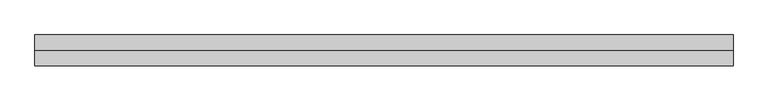
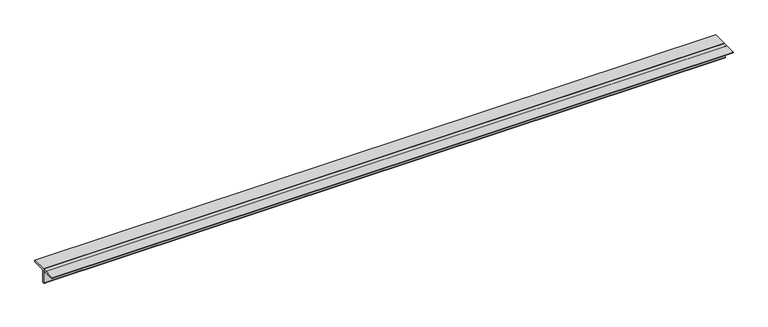
"""IFC4 building model written with IfcOpenShell, lengths in millimetres: member geometry, Steel Framing_2Ls_KS : H_SB_AR_S02_2Ls-100x100x10_VBR1."""

from ifc_helpers import new_model, si_unit, point, frame, frame_2d, origin, place, context, project, spatial, polyline, circle_curve, trimmed, segment, composite_curve, outline, extrude, source, transform, mapped, element, save


def member_e33f7588(model_context):
    return source(origin(), model_context, "Body", "SweptSolid", [
        extrude(outline(composite_curve([segment(polyline([(0.0, 28.2), (100.0, 28.2)]), True, "CONTINUOUS"), segment(trimmed(circle_curve(frame_2d((90.0, 28.2)), 10.0), [point((100.0, 28.2))], [point((90.0, 18.2))], False, "CARTESIAN"), True, "CONTINUOUS"), segment(polyline([(90.0, 18.2), (20.0, 18.2)]), True, "CONTINUOUS"), segment(trimmed(circle_curve(frame_2d((20.0, 8.2)), 10.0), [point((20.0, 18.2))], [point((10.0, 8.2))], True, "CARTESIAN"), True, "CONTINUOUS"), segment(polyline([(10.0, 8.2), (10.0, -61.8)]), True, "CONTINUOUS"), segment(trimmed(circle_curve(frame_2d((0.0, -61.8)), 10.0), [point((10.0, -61.8))], [point((0.0, -71.8))], False, "CARTESIAN"), True, "CONTINUOUS"), segment(polyline([(0.0, -71.8), (0.0, 28.2)]), True, "CONTINUOUS")], self_intersect=False)), frame((-2479.1576866, 0.0, 0.0), z_axis=(1.0, 0.0, 0.0), x_axis=(0.0, 1.0, 0.0)), (0.0, 0.0, 1.0), 4551.278999),
        extrude(outline(composite_curve([segment(polyline([(0.0, 28.2), (0.0, -71.8)]), True, "CONTINUOUS"), segment(trimmed(circle_curve(frame_2d((0.0, -61.8)), 10.0), [point((0.0, -71.8))], [point((-10.0, -61.8))], False, "CARTESIAN"), True, "CONTINUOUS"), segment(polyline([(-10.0, -61.8), (-10.0, 8.2)]), True, "CONTINUOUS"), segment(trimmed(circle_curve(frame_2d((-20.0, 8.2)), 10.0), [point((-10.0, 8.2))], [point((-20.0, 18.2))], True, "CARTESIAN"), True, "CONTINUOUS"), segment(polyline([(-20.0, 18.2), (-90.0, 18.2)]), True, "CONTINUOUS"), segment(trimmed(circle_curve(frame_2d((-90.0, 28.2)), 10.0), [point((-90.0, 18.2))], [point((-100.0, 28.2))], False, "CARTESIAN"), True, "CONTINUOUS"), segment(polyline([(-100.0, 28.2), (0.0, 28.2)]), True, "CONTINUOUS")], self_intersect=False)), frame((-2479.1576866, 0.0, 0.0), z_axis=(1.0, 0.0, 0.0), x_axis=(0.0, 1.0, 0.0)), (0.0, 0.0, 1.0), 4551.278999),
    ])


if __name__ == "__main__":
    model = new_model("IFC4")
    model_context = context("Model", 3, world=origin())
    ifc_project = project(units=[si_unit("LENGTHUNIT", "METRE", prefix="MILLI")], contexts=[model_context])
    site = spatial("IfcSite", under=ifc_project)
    building = spatial("IfcBuilding", under=site)
    placement = place(None, origin())
    member_shape = member_e33f7588(model_context)
    element("IfcMember", 1, ObjectType="Steel Framing_2Ls_KS : H_SB_AR_S02_2Ls-100x100x10_VBR1", at=placement, inside=building, context=model_context, shape_type="MappedRepresentation", body=[
        mapped(member_shape, transform((0.0, 0.0, 0.0), x_axis=(1.0, 0.0, 0.0), y_axis=(0.0, 1.0, 0.0), z_axis=(0.0, 0.0, 1.0))),
    ])
    save(model, "model.ifc")

# Revit data of these elements
# Type "Steel Framing_2Ls_KS : H_SB_AR_S02_2Ls-100x100x10_VBR1"
#   Type Comments = "MAIN"
#   Type Mark = "VBR1"
#   H_SectionID = "2Ls-100x100x10"
#   Assembly Code = "B10"
#   Legs = "LLBB"
#   H_Ratio for Additional Steel Plate = 0.2
#   W = 0
#   Perimeter = 0.80 m²/m
#   Nominal Weight = 29.80 kgf/m
#   Length [instance default] = 1524 mm
#   Space = 0 mm
#   b = 100 mm
#   d = 100 mm
#   t = 10 mm
#   y = 28.2 mm
#   A = 0.0038 m²
#   Structural Material [instance default] = Steel, 45-345
# Element 1 (IfcMember, "Steel Framing_2Ls_KS : H_SB_AR_S02_2Ls-100x100x10_VBR1")
#   Materials on its faces: "Steel, 45-345"
# Materials
#   "Steel, 45-345": class "Metal", colour RGB 189 187 185, transparency 0, Description = "Steel 345 MPa", Cost = 0
